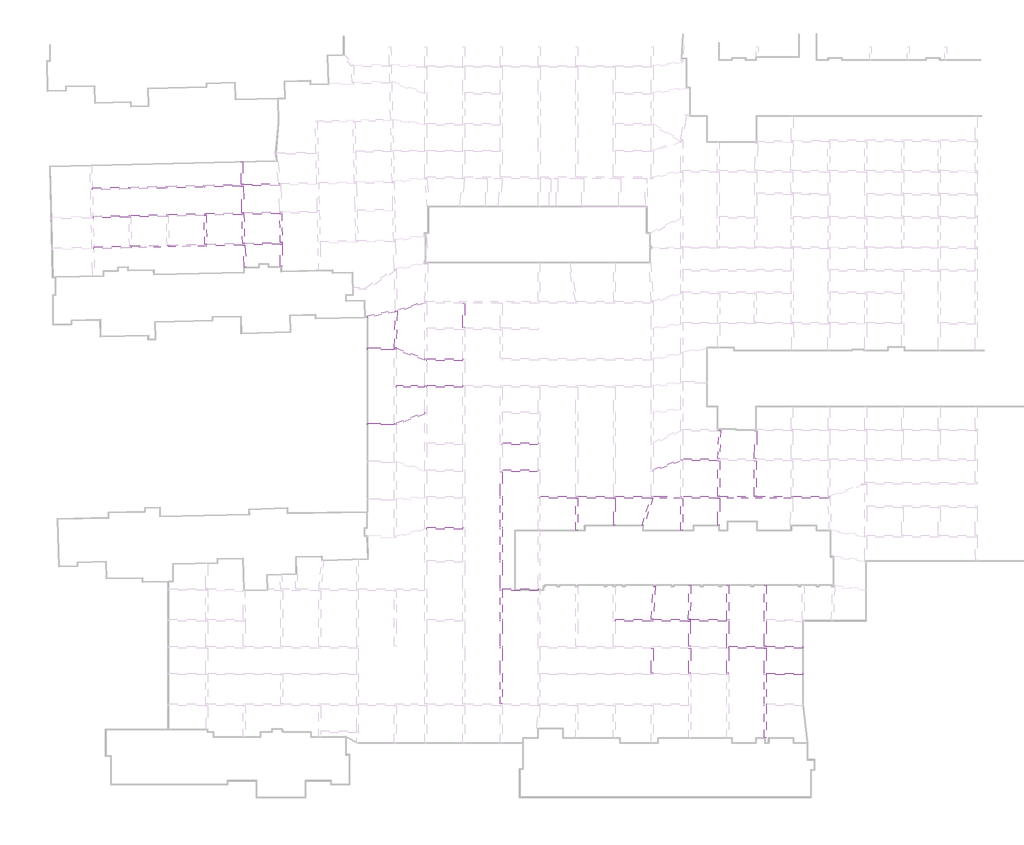
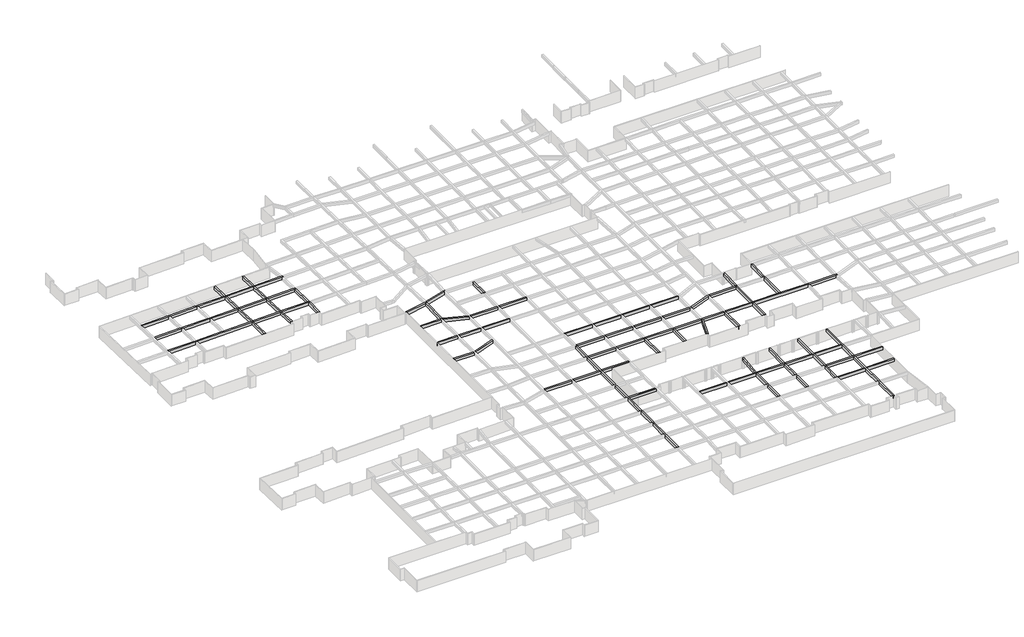
# One storey, part 10 of 20: 51 beams.
"""IFC4 building model written with IfcOpenShell, lengths in millimetres."""

import ifcopenshell
import ifcopenshell.guid

model = None  # the IFC model being written
_history = None  # IfcOwnerHistory: only IFC2X3 demands one
_inside = {}  # id of a spatial element -> (the spatial element, [elements in it])
_under = {}  # id of a project, library or spatial element -> (it, [spatial elements below it])
_declared = {}  # id of a project -> (the project, [libraries it declares])
_typed = {}  # id of a type object -> (the type object, [elements of that type])
_made_of = {}  # id of a material, layer set ... -> (it, [elements and type objects made of it])


def new_model(schema):
    """Start an empty IFC model of exactly this schema.

    Asked for "IFC4X3", IfcOpenShell would pick the latest addendum, in which some entities
    have other attributes; the version numbers below select the first issue.
    IFC2X3 requires an IfcOwnerHistory on every rooted entity: one is made here for all.
    """
    global model, _history
    if schema == "IFC4X3":
        model = ifcopenshell.file(schema_version=(4, 3, 0, 0))
    else:
        model = ifcopenshell.file(schema=schema)
    _inside.clear()
    _under.clear()
    _declared.clear()
    _typed.clear()
    _made_of.clear()
    _history = None
    if model.schema == "IFC2X3":
        org = make("IfcOrganization", Name="unknown")
        user = make(
            "IfcPersonAndOrganization",
            ThePerson=make("IfcPerson", FamilyName="unknown"),
            TheOrganization=org,
        )
        app = make(
            "IfcApplication",
            ApplicationDeveloper=org,
            Version="unknown",
            ApplicationFullName="unknown",
            ApplicationIdentifier="unknown",
        )
        _history = make(
            "IfcOwnerHistory",
            OwningUser=user,
            OwningApplication=app,
            ChangeAction="ADDED",
            CreationDate=0,
        )
    return model


def make(cls, **values):
    """One entity of the class cls with the attributes given. An attribute that is None is left unset."""
    return model.create_entity(
        cls, **{name: value for name, value in values.items() if value is not None}
    )


def rooted(cls, **values):
    """An entity with a GlobalId (a new one), such as an element, a storey or a relation."""
    return make(cls, GlobalId=ifcopenshell.guid.new(), OwnerHistory=_history, **values)


def si_unit(unit_type, name, prefix=None):
    """IfcSIUnit, for example si_unit("LENGTHUNIT", "METRE", prefix="MILLI")."""
    return make("IfcSIUnit", UnitType=unit_type, Prefix=prefix, Name=name)


def assignment(units):
    """IfcUnitAssignment: the units of a project."""
    return None if units is None else make("IfcUnitAssignment", Units=units)


def point(xyz):
    """IfcCartesianPoint."""
    return None if xyz is None else make("IfcCartesianPoint", Coordinates=xyz)


def direction(xyz):
    """IfcDirection."""
    return None if xyz is None else make("IfcDirection", DirectionRatios=xyz)


def frame(location, z_axis=None, x_axis=None):
    """IfcAxis2Placement3D, a coordinate frame: its origin and axes. An axis left out is left unset."""
    return make(
        "IfcAxis2Placement3D",
        Location=point(location),
        Axis=direction(z_axis),
        RefDirection=direction(x_axis),
    )


def origin():
    """The frame at (0, 0, 0) with its axes left unset."""
    return frame((0.0, 0.0, 0.0))


def place(relative_to, where):
    """IfcLocalPlacement: puts the frame where relative to a parent placement (None: the world)."""
    return make(
        "IfcLocalPlacement", PlacementRelTo=relative_to, RelativePlacement=where
    )


def context(
    kind, dimensions, precision=None, world=None, true_north=None, identifier=None
):
    """IfcGeometricRepresentationContext, for example the 3D "Model" context."""
    return make(
        "IfcGeometricRepresentationContext",
        ContextIdentifier=identifier,
        ContextType=kind,
        CoordinateSpaceDimension=dimensions,
        Precision=precision,
        WorldCoordinateSystem=world,
        TrueNorth=true_north,
    )


def project(units=None, contexts=None):
    """IfcProject with its units and contexts."""
    return rooted(
        "IfcProject",
        Name="project",
        RepresentationContexts=contexts,
        UnitsInContext=assignment(units),
    )


def spatial(cls, under=None, at=None, **own):
    """A site, building, storey or space (cls), placed at a placement, below another one or the project."""
    s = rooted(cls, ObjectPlacement=at, **own)
    if under is not None:
        _under.setdefault(under.id(), (under, []))[1].append(s)
    return s


def polyline(points):
    """IfcPolyline through the points."""
    return make("IfcPolyline", Points=[point(p) for p in points])


def outline(outer, holes=None, kind="AREA"):
    """IfcArbitraryClosedProfileDef: a profile drawn as a closed curve; with holes, ...WithVoids."""
    if holes is None:
        return make("IfcArbitraryClosedProfileDef", ProfileType=kind, OuterCurve=outer)
    return make(
        "IfcArbitraryProfileDefWithVoids",
        ProfileType=kind,
        OuterCurve=outer,
        InnerCurves=holes,
    )


def extrude(swept, where, along, depth):
    """IfcExtrudedAreaSolid: the profile swept, set in the frame where, extruded along a direction by depth."""
    return make(
        "IfcExtrudedAreaSolid",
        SweptArea=swept,
        Position=where,
        ExtrudedDirection=direction(along),
        Depth=depth,
    )


def faces_of(points, faces, orient=None, outer=None):
    """IfcFace entities. A face is a list of loops; a loop is a list of indices into points, from 0.

    orient and outer hold one flag for each loop. By default every Orientation is true, the
    first loop of a face is its IfcFaceOuterBound and the others are IfcFaceBound.
    """
    made = []
    for i, loops in enumerate(faces):
        bounds = []
        for j, loop in enumerate(loops):
            is_outer = j == 0 if outer is None else outer[i][j]
            bounds.append(
                make(
                    "IfcFaceOuterBound" if is_outer else "IfcFaceBound",
                    Bound=make("IfcPolyLoop", Polygon=[points[k] for k in loop]),
                    Orientation=True if orient is None else orient[i][j],
                )
            )
        made.append(make("IfcFace", Bounds=bounds))
    return made


def faceted_brep(points, faces, orient=None, outer=None, voids=None):
    """IfcFacetedBrep: a solid bounded by flat faces; with voids (closed shells), ...WithVoids."""
    shared = [point(p) for p in points]
    hull = make("IfcClosedShell", CfsFaces=faces_of(shared, faces, orient, outer))
    if voids is None:
        return make("IfcFacetedBrep", Outer=hull)
    return make(
        "IfcFacetedBrepWithVoids",
        Outer=hull,
        Voids=[
            make(cls, CfsFaces=faces_of(shared, fs, o, b)) for cls, fs, o, b in voids
        ],
    )


def shape(context_of_items, identifier, shape_type, items):
    """IfcShapeRepresentation: the items that make up one representation, for example the "Body"."""
    return make(
        "IfcShapeRepresentation",
        ContextOfItems=context_of_items,
        RepresentationIdentifier=identifier,
        RepresentationType=shape_type,
        Items=items,
    )


def made_of(thing, what):
    """Note that an element or type object is made of a material, layer set ...; save() writes the relation."""
    if what is not None:
        _made_of.setdefault(what.id(), (what, []))[1].append(thing)
    return thing


def element(
    cls,
    number,
    at=None,
    inside=None,
    cuts=None,
    type_object=None,
    material=None,
    context=None,
    identifier="Body",
    shape_type=None,
    held_by="IfcProductDefinitionShape",
    body=None,
    shapes=None,
    **own,
):
    """One element of the class cls, such as IfcWall. Its Tag is "e" and its number.

    at: its placement. inside: the storey or other place that contains it. cuts: it is an
    opening in that element (IfcRelVoidsElement). A single representation is given by context,
    identifier, shape_type and body (its items); several are given by shapes. held_by: the class
    of the entity that holds the representations. save() writes the other relations.
    """
    e = rooted(cls, Tag="e%d" % number, ObjectPlacement=at, **own)
    if body is not None:
        shapes = [shape(context, identifier, shape_type, body)]
    if shapes is not None:
        e.Representation = make(held_by, Representations=shapes)
    if inside is not None:
        _inside.setdefault(inside.id(), (inside, []))[1].append(e)
    if cuts is not None:
        rooted(
            "IfcRelVoidsElement", RelatingBuildingElement=cuts, RelatedOpeningElement=e
        )
    if type_object is not None:
        _typed.setdefault(type_object.id(), (type_object, []))[1].append(e)
    return made_of(e, material)


def aggregate(whole, parts):
    """IfcRelAggregates: a whole, such as a stair, and the parts it consists of."""
    return rooted("IfcRelAggregates", RelatingObject=whole, RelatedObjects=parts)


def save(model, path):
    """Write the relations noted so far, then the file.

    IfcRelAggregates (storeys below a building ...), IfcRelContainedInSpatialStructure (elements
    in a storey), IfcRelDefinesByType, IfcRelAssociatesMaterial and IfcRelDeclares: one each for
    every whole, place, type object, material and project.
    """
    for whole, parts in _under.values():
        aggregate(whole, parts)
    for where, things in _inside.values():
        rooted(
            "IfcRelContainedInSpatialStructure",
            RelatedElements=things,
            RelatingStructure=where,
        )
    for kind, things in _typed.values():
        rooted("IfcRelDefinesByType", RelatedObjects=things, RelatingType=kind)
    for what, things in _made_of.values():
        rooted("IfcRelAssociatesMaterial", RelatedObjects=things, RelatingMaterial=what)
    for by, libraries in _declared.values():
        rooted("IfcRelDeclares", RelatingContext=by, RelatedDefinitions=libraries)
    model.write(path)


model = new_model("IFC4")

# Units and contexts
model_context = context("Model", 3, world=origin())
ifc_project = project(units=[si_unit("LENGTHUNIT", "METRE", prefix="MILLI")], contexts=[model_context])

# Site, building, storey
site = spatial("IfcSite", under=ifc_project)
building = spatial("IfcBuilding", under=site)
storey = spatial("IfcBuildingStorey", under=building, Name="户型图", Elevation=0.0)

# Beams
placement = place(None, origin())
element("IfcBeam", 1, ObjectType="混凝土 - 矩形梁 : KL_beam", at=placement, inside=storey, context=model_context, shape_type="SweptSolid", body=[
    extrude(outline(polyline([(102845.0, 57619.9584924), (102845.0, 58045.6296013), (108750.0, 60194.8738347), (108750.0, 59769.2027257), (102845.0, 57619.9584924)])), frame((0.0, 0.0, 2500.0), z_axis=(0.0, 0.0, 1.0), x_axis=(1.0, 0.0, 0.0)), (0.0, 0.0, 1.0), 800.0),
])
element("IfcBeam", 2, ObjectType="混凝土 - 矩形梁 : KL_beam", at=placement, inside=storey, context=model_context, shape_type="SweptSolid", body=[
    extrude(outline(polyline([(102445.0, 63683.0), (102445.0, 63283.0), (94850.0, 63283.0), (94850.0, 63683.0), (102445.0, 63683.0)])), frame((0.0, 0.0, 2500.0), z_axis=(0.0, 0.0, 1.0), x_axis=(1.0, 0.0, 0.0)), (0.0, 0.0, 1.0), 800.0),
    extrude(outline(polyline([(70850.0, 63283.0), (70850.0, 63683.0), (78450.0, 63683.0), (78450.0, 63283.0), (70850.0, 63283.0)])), frame((0.0, 0.0, 2500.0), z_axis=(0.0, 0.0, 1.0), x_axis=(1.0, 0.0, 0.0)), (0.0, 0.0, 1.0), 800.0),
    extrude(outline(polyline([(78850.0, 63283.0), (78850.0, 63683.0), (86450.0, 63683.0), (86450.0, 63283.0), (78850.0, 63283.0)])), frame((0.0, 0.0, 2500.0), z_axis=(0.0, 0.0, 1.0), x_axis=(1.0, 0.0, 0.0)), (0.0, 0.0, 1.0), 800.0),
    extrude(outline(polyline([(86850.0, 63283.0), (86850.0, 63683.0), (94450.0, 63683.0), (94450.0, 63283.0), (86850.0, 63283.0)])), frame((0.0, 0.0, 2500.0), z_axis=(0.0, 0.0, 1.0), x_axis=(1.0, 0.0, 0.0)), (0.0, 0.0, 1.0), 800.0),
])
element("IfcBeam", 3, ObjectType="混凝土 - 矩形梁 : KL_beam", at=placement, inside=storey, context=model_context, shape_type="SweptSolid", body=[
    extrude(outline(polyline([(102445.0, 57960.0), (102445.0, 57560.0), (94850.0, 57560.0), (94850.0, 57960.0), (102445.0, 57960.0)])), frame((0.0, 0.0, 2500.0), z_axis=(0.0, 0.0, 1.0), x_axis=(1.0, 0.0, 0.0)), (0.0, 0.0, 1.0), 800.0),
    extrude(outline(polyline([(70850.0, 57560.0), (70850.0, 57960.0), (78450.0, 57960.0), (78450.0, 57560.0), (70850.0, 57560.0)])), frame((0.0, 0.0, 2500.0), z_axis=(0.0, 0.0, 1.0), x_axis=(1.0, 0.0, 0.0)), (0.0, 0.0, 1.0), 800.0),
    extrude(outline(polyline([(78850.0, 57560.0), (78850.0, 57960.0), (86450.0, 57960.0), (86450.0, 57560.0), (78850.0, 57560.0)])), frame((0.0, 0.0, 2500.0), z_axis=(0.0, 0.0, 1.0), x_axis=(1.0, 0.0, 0.0)), (0.0, 0.0, 1.0), 800.0),
    extrude(outline(polyline([(86850.0, 57560.0), (86850.0, 57960.0), (94450.0, 57960.0), (94450.0, 57560.0), (86850.0, 57560.0)])), frame((0.0, 0.0, 2500.0), z_axis=(0.0, 0.0, 1.0), x_axis=(1.0, 0.0, 0.0)), (0.0, 0.0, 1.0), 800.0),
])
element("IfcBeam", 4, ObjectType="混凝土 - 矩形梁 : KL_beam", at=placement, inside=storey, context=model_context, shape_type="Brep", body=[
    faceted_brep([(108750.0, 51965.0, 3300.0), (108750.0, 52365.0, 3300.0), (102845.0, 52365.0, 3300.0), (102445.0, 52365.0, 3300.0), (94850.0, 52365.0, 3300.0), (94450.0, 52365.0, 3300.0), (86850.0, 52365.0, 3300.0), (86450.0, 52365.0, 3300.0), (78850.0, 52365.0, 3300.0), (78850.0, 51965.0, 3300.0), (86450.0, 51965.0, 3300.0), (86850.0, 51965.0, 3300.0), (94450.0, 51965.0, 3300.0), (94850.0, 51965.0, 3300.0), (102369.758159, 51965.0, 3300.0), (102790.3267419, 51965.0, 3300.0), (108750.0, 52365.0, 2500.0), (102845.0, 52365.0, 2500.0), (102445.0, 52365.0, 2500.0), (94850.0, 52365.0, 2500.0), (94450.0, 52365.0, 2500.0), (86850.0, 52365.0, 2500.0), (86450.0, 52365.0, 2500.0), (78850.0, 52365.0, 2500.0), (108750.0, 51965.0, 2500.0), (102790.3267419, 51965.0, 2500.0), (102369.758159, 51965.0, 2500.0), (94850.0, 51965.0, 2500.0), (94450.0, 51965.0, 2500.0), (86850.0, 51965.0, 2500.0), (86450.0, 51965.0, 2500.0), (78850.0, 51965.0, 2500.0)], [[[0, 1, 2, 3, 4, 5, 6, 7, 8, 9, 10, 11, 12, 13, 14, 15]], [[1, 16, 17, 18, 19, 20, 21, 22, 23, 8, 7, 6, 5, 4, 3, 2]], [[16, 24, 25, 26, 27, 28, 29, 30, 31, 23, 22, 21, 20, 19, 18, 17]], [[24, 0, 15, 14, 13, 12, 11, 10, 9, 31, 30, 29, 28, 27, 26, 25]], [[1, 0, 24, 16]], [[9, 8, 23, 31]]]),
    faceted_brep([(78450.0, 52365.0, 3300.0), (78450.0, 51965.0, 3300.0), (78450.0, 51965.0, 2500.0), (78450.0, 52365.0, 2500.0), (70850.0, 52365.0, 3300.0), (70850.0, 51965.0, 3300.0), (70850.0, 52365.0, 2500.0), (70850.0, 51965.0, 2500.0)], [[[0, 1, 2, 3]], [[1, 0, 4, 5]], [[0, 3, 6, 4]], [[3, 2, 7, 6]], [[2, 1, 5, 7]], [[5, 4, 6, 7]]]),
])
element("IfcBeam", 5, ObjectType="混凝土 - 矩形梁 : KL_beam", at=placement, inside=storey, context=model_context, shape_type="Brep", body=[
    faceted_brep([(70850.0, 57560.0, 3300.0), (70450.0, 57560.0, 3300.0), (70450.0, 52365.0, 3300.0), (70450.0, 51965.0, 3300.0), (70450.0, 45760.0, 3300.0), (70450.0, 45360.0, 3300.0), (70450.0, 38790.0, 3300.0), (70450.0, 38390.0, 3300.0), (70450.0, 32740.0, 3300.0), (70450.0, 32340.0, 3300.0), (70450.0, 26240.0, 3300.0), (70450.0, 25840.0, 3300.0), (70450.0, 20540.0, 3300.0), (70450.0, 20140.0, 3300.0), (70450.0, 14840.0, 3300.0), (70450.0, 14440.0, 3300.0), (70450.0, 8340.0, 3300.0), (70850.0, 8340.0, 3300.0), (70850.0, 14440.0, 3300.0), (70850.0, 14840.0, 3300.0), (70850.0, 20140.0, 3300.0), (70850.0, 20540.0, 3300.0), (70850.0, 25840.0, 3300.0), (70850.0, 26240.0, 3300.0), (70850.0, 32340.0, 3300.0), (70850.0, 32740.0, 3300.0), (70850.0, 38390.0, 3300.0), (70850.0, 38790.0, 3300.0), (70850.0, 45360.0, 3300.0), (70850.0, 45760.0, 3300.0), (70850.0, 51965.0, 3300.0), (70850.0, 52365.0, 3300.0), (70450.0, 57560.0, 2500.0), (70450.0, 52365.0, 2500.0), (70450.0, 51965.0, 2500.0), (70450.0, 45760.0, 2500.0), (70450.0, 45360.0, 2500.0), (70450.0, 38790.0, 2500.0), (70450.0, 38390.0, 2500.0), (70450.0, 32740.0, 2500.0), (70450.0, 32340.0, 2500.0), (70450.0, 26240.0, 2500.0), (70450.0, 25840.0, 2500.0), (70450.0, 20540.0, 2500.0), (70450.0, 20140.0, 2500.0), (70450.0, 14840.0, 2500.0), (70450.0, 14440.0, 2500.0), (70450.0, 8340.0, 2500.0), (70850.0, 57560.0, 2500.0), (70850.0, 52365.0, 2500.0), (70850.0, 51965.0, 2500.0), (70850.0, 45760.0, 2500.0), (70850.0, 45360.0, 2500.0), (70850.0, 38790.0, 2500.0), (70850.0, 38390.0, 2500.0), (70850.0, 32740.0, 2500.0), (70850.0, 32340.0, 2500.0), (70850.0, 26240.0, 2500.0), (70850.0, 25840.0, 2500.0), (70850.0, 20540.0, 2500.0), (70850.0, 20140.0, 2500.0), (70850.0, 14840.0, 2500.0), (70850.0, 14440.0, 2500.0), (70850.0, 8340.0, 2500.0)], [[[0, 1, 2, 3, 4, 5, 6, 7, 8, 9, 10, 11, 12, 13, 14, 15, 16, 17, 18, 19, 20, 21, 22, 23, 24, 25, 26, 27, 28, 29, 30, 31]], [[1, 32, 33, 34, 35, 36, 37, 38, 39, 40, 41, 42, 43, 44, 45, 46, 47, 16, 15, 14, 13, 12, 11, 10, 9, 8, 7, 6, 5, 4, 3, 2]], [[32, 48, 49, 50, 51, 52, 53, 54, 55, 56, 57, 58, 59, 60, 61, 62, 63, 47, 46, 45, 44, 43, 42, 41, 40, 39, 38, 37, 36, 35, 34, 33]], [[48, 0, 31, 30, 29, 28, 27, 26, 25, 24, 23, 22, 21, 20, 19, 18, 17, 63, 62, 61, 60, 59, 58, 57, 56, 55, 54, 53, 52, 51, 50, 49]], [[1, 0, 48, 32]], [[17, 16, 47, 63]]]),
])
element("IfcBeam", 6, ObjectType="混凝土 - 矩形梁 : KL_beam", at=placement, inside=storey, context=model_context, shape_type="SweptSolid", body=[
    extrude(outline(polyline([(62450.0, 93310.0), (62850.0, 93310.0), (62850.0, 88060.0), (62450.0, 88060.0), (62450.0, 93310.0)])), frame((0.0, 0.0, 2500.0), z_axis=(0.0, 0.0, 1.0), x_axis=(1.0, 0.0, 0.0)), (0.0, 0.0, 1.0), 800.0),
])
element("IfcBeam", 7, ObjectType="混凝土 - 矩形梁 : KL_beam", at=placement, inside=storey, context=model_context, shape_type="SweptSolid", body=[
    extrude(outline(polyline([(54850.0, 81110.0), (54850.0, 81510.0), (62450.0, 81510.0), (62450.0, 81110.0), (54850.0, 81110.0)])), frame((0.0, 0.0, 2500.0), z_axis=(0.0, 0.0, 1.0), x_axis=(1.0, 0.0, 0.0)), (0.0, 0.0, 1.0), 800.0),
    extrude(outline(polyline([(70450.0, 81510.0), (70450.0, 81110.0), (62850.0, 81110.0), (62850.0, 81510.0), (70450.0, 81510.0)])), frame((0.0, 0.0, 2500.0), z_axis=(0.0, 0.0, 1.0), x_axis=(1.0, 0.0, 0.0)), (0.0, 0.0, 1.0), 800.0),
])
element("IfcBeam", 8, ObjectType="混凝土 - 矩形梁 : KL_beam", at=placement, inside=storey, context=model_context, shape_type="SweptSolid", body=[
    extrude(outline(polyline([(62450.0, 75860.0), (62450.0, 75460.0), (54850.0, 75460.0), (54850.0, 75860.0), (62450.0, 75860.0)])), frame((0.0, 0.0, 2500.0), z_axis=(0.0, 0.0, 1.0), x_axis=(1.0, 0.0, 0.0)), (0.0, 0.0, 1.0), 800.0),
])
element("IfcBeam", 9, ObjectType="混凝土 - 矩形梁 : KL_beam", at=placement, inside=storey, context=model_context, shape_type="SweptSolid", body=[
    extrude(outline(polyline([(78450.0, 45760.0), (78450.0, 45360.0), (70850.0, 45360.0), (70850.0, 45760.0), (78450.0, 45760.0)])), frame((0.0, 0.0, 2500.0), z_axis=(0.0, 0.0, 1.0), x_axis=(1.0, 0.0, 0.0)), (0.0, 0.0, 1.0), 800.0),
    extrude(outline(polyline([(54850.0, 45360.0), (54850.0, 45760.0), (62450.0, 45760.0), (62450.0, 45360.0), (54850.0, 45360.0)])), frame((0.0, 0.0, 2500.0), z_axis=(0.0, 0.0, 1.0), x_axis=(1.0, 0.0, 0.0)), (0.0, 0.0, 1.0), 800.0),
    extrude(outline(polyline([(70450.0, 45760.0), (70450.0, 45360.0), (62850.0, 45360.0), (62850.0, 45760.0), (70450.0, 45760.0)])), frame((0.0, 0.0, 2500.0), z_axis=(0.0, 0.0, 1.0), x_axis=(1.0, 0.0, 0.0)), (0.0, 0.0, 1.0), 800.0),
])
element("IfcBeam", 10, ObjectType="混凝土 - 矩形梁 : KL_beam", at=placement, inside=storey, context=model_context, shape_type="Brep", body=[
    faceted_brep([(110728.5214786, 25840.0, 3300.0), (110725.0304656, 26040.0, 3300.0), (110721.5394526, 26240.0, 3300.0), (110328.4605474, 26240.0, 3300.0), (102848.6320497, 26240.0, 3300.0), (102447.6345431, 26240.0, 3300.0), (94845.0, 26240.0, 3300.0), (94845.0, 25840.0, 3300.0), (102434.0, 25840.0, 3300.0), (102834.0, 25840.0, 3300.0), (110328.4605474, 25840.0, 3300.0), (110728.5214786, 25840.0, 2500.0), (94845.0, 25840.0, 2500.0), (102434.0, 25840.0, 2500.0), (102834.0, 25840.0, 2500.0), (110328.4605474, 25840.0, 2500.0), (110721.5394526, 26240.0, 2500.0), (110725.0304656, 26040.0, 2500.0), (94845.0, 26240.0, 2500.0), (102447.6345431, 26240.0, 2500.0), (102848.6320497, 26240.0, 2500.0), (110328.4605474, 26240.0, 2500.0)], [[[0, 1, 2, 3, 4, 5, 6, 7, 8, 9, 10]], [[11, 0, 10, 9, 8, 7, 12, 13, 14, 15]], [[16, 17, 11, 15, 14, 13, 12, 18, 19, 20, 21]], [[2, 16, 21, 20, 19, 18, 6, 5, 4, 3]], [[7, 6, 18, 12]], [[2, 1, 0, 11, 17, 16]]]),
    faceted_brep([(86850.0, 25840.0, 3300.0), (86850.0, 26240.0, 3300.0), (86850.0, 26240.0, 2500.0), (86850.0, 25840.0, 2500.0), (94445.0, 26240.0, 3300.0), (94445.0, 25840.0, 3300.0), (94445.0, 25840.0, 2500.0), (94445.0, 26240.0, 2500.0)], [[[0, 1, 2, 3]], [[4, 5, 6, 7]], [[1, 0, 5, 4]], [[0, 3, 6, 5]], [[3, 2, 7, 6]], [[2, 1, 4, 7]]]),
])
element("IfcBeam", 11, ObjectType="混凝土 - 矩形梁 : KL_beam", at=placement, inside=storey, context=model_context, shape_type="SweptSolid", body=[
    extrude(outline(polyline([(102434.0, 25840.0), (102834.0, 25840.0), (102834.0, 20540.0), (102434.0, 20540.0), (102434.0, 25840.0)])), frame((0.0, 0.0, 2500.0), z_axis=(0.0, 0.0, 1.0), x_axis=(1.0, 0.0, 0.0)), (0.0, 0.0, 1.0), 800.0),
    extrude(outline(polyline([(102834.0, 14840.0), (102434.0, 14840.0), (102434.0, 20140.0), (102834.0, 20140.0), (102834.0, 14840.0)])), frame((0.0, 0.0, 2500.0), z_axis=(0.0, 0.0, 1.0), x_axis=(1.0, 0.0, 0.0)), (0.0, 0.0, 1.0), 800.0),
])
element("IfcBeam", 12, ObjectType="混凝土 - 矩形梁 : KL_beam", at=placement, inside=storey, context=model_context, shape_type="SweptSolid", body=[
    extrude(outline(polyline([(110328.4605474, 25840.0), (110728.5214786, 25840.0), (110821.0333227, 20540.0), (110420.9723915, 20540.0), (110328.4605474, 25840.0)])), frame((0.0, 0.0, 2500.0), z_axis=(0.0, 0.0, 1.0), x_axis=(1.0, 0.0, 0.0)), (0.0, 0.0, 1.0), 800.0),
])
element("IfcBeam", 13, ObjectType="混凝土 - 矩形梁 : KL_beam", at=placement, inside=storey, context=model_context, shape_type="SweptSolid", body=[
    extrude(outline(polyline([(110824.4938701, 14840.0), (110424.4938701, 14840.0), (110424.4938701, 20140.0), (110824.4938701, 20140.0), (110824.4938701, 14840.0)])), frame((0.0, 0.0, 2500.0), z_axis=(0.0, 0.0, 1.0), x_axis=(1.0, 0.0, 0.0)), (0.0, 0.0, 1.0), 800.0),
])
element("IfcBeam", 14, ObjectType="混凝土 - 矩形梁 : KL_beam", at=placement, inside=storey, context=model_context, shape_type="Brep", body=[
    faceted_brep([(118450.0, 33507.0, 3300.0), (118850.0, 33507.0, 3300.0), (118850.0, 33507.0, 2500.0), (118450.0, 33507.0, 2500.0), (118450.0, 26240.0, 3300.0), (118450.0, 25840.0, 3300.0), (118450.0, 20540.0, 3300.0), (118450.0, 20140.0, 3300.0), (118450.0, 14840.0, 3300.0), (118850.0, 14840.0, 3300.0), (118850.0, 20140.0, 3300.0), (118850.0, 20540.0, 3300.0), (118850.0, 25840.0, 3300.0), (118850.0, 26240.0, 3300.0), (118850.0, 14840.0, 2500.0), (118850.0, 20140.0, 2500.0), (118850.0, 20540.0, 2500.0), (118850.0, 25840.0, 2500.0), (118850.0, 26240.0, 2500.0), (118450.0, 14840.0, 2500.0), (118450.0, 20140.0, 2500.0), (118450.0, 20540.0, 2500.0), (118450.0, 25840.0, 2500.0), (118450.0, 26240.0, 2500.0)], [[[0, 1, 2, 3]], [[1, 0, 4, 5, 6, 7, 8, 9, 10, 11, 12, 13]], [[2, 1, 13, 12, 11, 10, 9, 14, 15, 16, 17, 18]], [[3, 2, 18, 17, 16, 15, 14, 19, 20, 21, 22, 23]], [[0, 3, 23, 22, 21, 20, 19, 8, 7, 6, 5, 4]], [[9, 8, 19, 14]]]),
])
element("IfcBeam", 15, ObjectType="混凝土 - 矩形梁 : KL_beam", at=placement, inside=storey, context=model_context, shape_type="Brep", body=[
    faceted_brep([(110454.5273167, 33462.3603793, 3300.0), (110854.4663948, 33455.3794168, 3300.0), (110854.4663948, 33455.3794168, 2500.0), (110454.5273167, 33462.3603793, 2500.0), (110328.4605474, 26240.0, 3300.0), (110721.5394526, 26240.0, 3300.0), (110725.0304656, 26040.0, 3300.0), (110728.5214786, 26240.0, 3300.0), (110725.0304656, 26040.0, 2500.0), (110728.5214786, 26240.0, 2500.0), (110721.5394526, 26240.0, 2500.0), (110328.4605474, 26240.0, 2500.0)], [[[0, 1, 2, 3]], [[1, 0, 4, 5, 6, 7]], [[2, 1, 7, 6, 8, 9]], [[3, 2, 9, 8, 10, 11]], [[0, 3, 11, 4]], [[10, 5, 4, 11]], [[5, 10, 8, 6]]]),
])
element("IfcBeam", 16, ObjectType="混凝土 - 矩形梁 : KL_beam", at=placement, inside=storey, context=model_context, shape_type="SweptSolid", body=[
    extrude(outline(polyline([(102944.4623549, 33270.6006236), (103343.4673297, 33242.4043457), (102848.6320497, 26240.0), (102447.6345431, 26240.0), (102944.4623549, 33270.6006236)])), frame((0.0, 0.0, 2500.0), z_axis=(0.0, 0.0, 1.0), x_axis=(1.0, 0.0, 0.0)), (0.0, 0.0, 1.0), 800.0),
])
element("IfcBeam", 17, ObjectType="混凝土 - 矩形梁 : KL_beam", at=placement, inside=storey, context=model_context, shape_type="SweptSolid", body=[
    extrude(outline(polyline([(110728.5214786, 25840.0), (110725.0304656, 26040.0), (110728.5214786, 26240.0), (118450.0, 26240.0), (118450.0, 25840.0), (110728.5214786, 25840.0)])), frame((0.0, 0.0, 2500.0), z_axis=(0.0, 0.0, 1.0), x_axis=(1.0, 0.0, 0.0)), (0.0, 0.0, 1.0), 800.0),
    extrude(outline(polyline([(118850.0, 25840.0), (118850.0, 26240.0), (126444.0, 26240.0), (126444.0, 25840.0), (118850.0, 25840.0)])), frame((0.0, 0.0, 2500.0), z_axis=(0.0, 0.0, 1.0), x_axis=(1.0, 0.0, 0.0)), (0.0, 0.0, 1.0), 800.0),
])
element("IfcBeam", 18, ObjectType="混凝土 - 矩形梁 : KL_beam", at=placement, inside=storey, context=model_context, shape_type="Brep", body=[
    faceted_brep([(126844.0, 33507.0, 3300.0), (126844.0, 33507.0, 2500.0), (126444.0, 33507.0, 2500.0), (126444.0, 33507.0, 3300.0), (126444.0, 26240.0, 3300.0), (126444.0, 25840.0, 3300.0), (126444.0, 20540.0, 3300.0), (126844.0, 20540.0, 3300.0), (126844.0, 25837.4184717, 3300.0), (126844.0, 26237.453407, 3300.0), (126444.0, 26240.0, 2500.0), (126444.0, 25840.0, 2500.0), (126444.0, 20540.0, 2500.0), (126844.0, 26237.453407, 2500.0), (126844.0, 25837.4184717, 2500.0), (126844.0, 20540.0, 2500.0)], [[[0, 1, 2, 3]], [[0, 3, 4, 5, 6, 7, 8, 9]], [[3, 2, 10, 11, 12, 6, 5, 4]], [[2, 1, 13, 14, 15, 12, 11, 10]], [[1, 0, 9, 8, 7, 15, 14, 13]], [[7, 6, 12, 15]]]),
])
element("IfcBeam", 19, ObjectType="混凝土 - 矩形梁 : KL_beam", at=placement, inside=storey, context=model_context, shape_type="Brep", body=[
    faceted_brep([(134623.3674306, 20540.0, 3300.0), (134623.3674306, 20140.0, 3300.0), (134623.3674306, 20140.0, 2500.0), (134623.3674306, 20540.0, 2500.0), (126844.0, 20540.0, 3300.0), (126444.0, 20540.0, 3300.0), (118850.0, 20540.0, 3300.0), (118850.0, 20140.0, 3300.0), (126444.0, 20140.0, 3300.0), (126844.0, 20140.0, 3300.0), (118850.0, 20140.0, 2500.0), (126444.0, 20140.0, 2500.0), (126844.0, 20140.0, 2500.0), (118850.0, 20540.0, 2500.0), (126444.0, 20540.0, 2500.0), (126844.0, 20540.0, 2500.0)], [[[0, 1, 2, 3]], [[1, 0, 4, 5, 6, 7, 8, 9]], [[2, 1, 9, 8, 7, 10, 11, 12]], [[3, 2, 12, 11, 10, 13, 14, 15]], [[0, 3, 15, 14, 13, 6, 5, 4]], [[7, 6, 13, 10]]]),
])
element("IfcBeam", 20, ObjectType="混凝土 - 矩形梁 : KL_beam", at=placement, inside=storey, context=model_context, shape_type="Brep", body=[
    faceted_brep([(126844.0, 1106.0, 3300.0), (126444.0, 1106.0, 3300.0), (126444.0, 1106.0, 2500.0), (126844.0, 1106.0, 2500.0), (126844.0, 7940.0, 3300.0), (126844.0, 8340.0, 3300.0), (126844.0, 14440.0, 3300.0), (126844.0, 14840.0, 3300.0), (126844.0, 20140.0, 3300.0), (126444.0, 20140.0, 3300.0), (126444.0, 14840.0, 3300.0), (126444.0, 14440.0, 3300.0), (126444.0, 8340.0, 3300.0), (126444.0, 7940.0, 3300.0), (126444.0, 20140.0, 2500.0), (126444.0, 14840.0, 2500.0), (126444.0, 14440.0, 2500.0), (126444.0, 8340.0, 2500.0), (126444.0, 7940.0, 2500.0), (126844.0, 20140.0, 2500.0), (126844.0, 14840.0, 2500.0), (126844.0, 14440.0, 2500.0), (126844.0, 8340.0, 2500.0), (126844.0, 7940.0, 2500.0)], [[[0, 1, 2, 3]], [[1, 0, 4, 5, 6, 7, 8, 9, 10, 11, 12, 13]], [[2, 1, 13, 12, 11, 10, 9, 14, 15, 16, 17, 18]], [[3, 2, 18, 17, 16, 15, 14, 19, 20, 21, 22, 23]], [[0, 3, 23, 22, 21, 20, 19, 8, 7, 6, 5, 4]], [[9, 8, 19, 14]]]),
])
element("IfcBeam", 21, ObjectType="混凝土 - 矩形梁 : KL_beam", at=placement, inside=storey, context=model_context, shape_type="SweptSolid", body=[
    extrude(outline(polyline([(134623.3674306, 14840.0), (134623.3674306, 14440.0), (126844.0, 14440.0), (126844.0, 14840.0), (134623.3674306, 14840.0)])), frame((0.0, 0.0, 2500.0), z_axis=(0.0, 0.0, 1.0), x_axis=(1.0, 0.0, 0.0)), (0.0, 0.0, 1.0), 800.0),
    extrude(outline(polyline([(118850.0, 14440.0), (118850.0, 14840.0), (126444.0, 14840.0), (126444.0, 14440.0), (118850.0, 14440.0)])), frame((0.0, 0.0, 2500.0), z_axis=(0.0, 0.0, 1.0), x_axis=(1.0, 0.0, 0.0)), (0.0, 0.0, 1.0), 800.0),
])
element("IfcBeam", 22, ObjectType="混凝土 - 矩形梁 : KL_beam", at=placement, inside=storey, context=model_context, shape_type="Brep", body=[
    faceted_brep([(48350.0, 83800.3620102, 3300.0), (48350.0, 83375.0226052, 3300.0), (54450.0, 81169.6379898, 3300.0), (54450.0, 81594.9773948, 3300.0), (48353.8968226, 83798.953159, 3300.0), (48350.0, 83375.0226052, 2500.0), (54450.0, 81169.6379898, 2500.0), (48350.0, 83800.3620102, 2500.0), (48353.8968226, 83798.953159, 2500.0), (54450.0, 81594.9773948, 2500.0)], [[[0, 1, 2, 3, 4]], [[1, 5, 6, 2]], [[5, 7, 8, 9, 6]], [[7, 0, 4, 3, 9, 8]], [[1, 0, 7, 5]], [[3, 2, 6, 9]]]),
])
element("IfcBeam", 23, ObjectType="混凝土 - 矩形梁 : KL_beam", at=placement, inside=storey, context=model_context, shape_type="SweptSolid", body=[
    extrude(outline(polyline([(42250.0, 75460.0), (42250.0, 75860.0), (47950.0, 75860.0), (47950.0, 75460.0), (42250.0, 75460.0)])), frame((0.0, 0.0, 2500.0), z_axis=(0.0, 0.0, 1.0), x_axis=(1.0, 0.0, 0.0)), (0.0, 0.0, 1.0), 800.0),
    extrude(outline(polyline([(54450.0, 75860.0), (54450.0, 75460.0), (48350.0, 75460.0), (48350.0, 75860.0), (54450.0, 75860.0)])), frame((0.0, 0.0, 2500.0), z_axis=(0.0, 0.0, 1.0), x_axis=(1.0, 0.0, 0.0)), (0.0, 0.0, 1.0), 800.0),
])
element("IfcBeam", 24, ObjectType="混凝土 - 矩形梁 : KL_beam", at=placement, inside=storey, context=model_context, shape_type="SweptSolid", body=[
    extrude(outline(polyline([(42250.0, 67460.0), (42250.0, 67860.0), (47950.0, 67860.0), (47950.0, 67460.0), (42250.0, 67460.0)])), frame((0.0, 0.0, 2500.0), z_axis=(0.0, 0.0, 1.0), x_axis=(1.0, 0.0, 0.0)), (0.0, 0.0, 1.0), 800.0),
])
element("IfcBeam", 25, ObjectType="混凝土 - 矩形梁 : KL_beam", at=placement, inside=storey, context=model_context, shape_type="SweptSolid", body=[
    extrude(outline(polyline([(54450.0, 70165.8480304), (54450.0, 69740.1769214), (48350.0, 67519.9584924), (48350.0, 67945.6296013), (54450.0, 70165.8480304)])), frame((0.0, 0.0, 2500.0), z_axis=(0.0, 0.0, 1.0), x_axis=(1.0, 0.0, 0.0)), (0.0, 0.0, 1.0), 800.0),
])
element("IfcBeam", 26, ObjectType="混凝土 - 矩形梁 : KL_beam", at=placement, inside=storey, context=model_context, shape_type="SweptSolid", body=[
    extrude(outline(polyline([(70850.0, 32340.0), (70850.0, 32740.0), (78450.0, 32740.0), (78450.0, 32340.0), (70850.0, 32340.0)])), frame((0.0, 0.0, 2500.0), z_axis=(0.0, 0.0, 1.0), x_axis=(1.0, 0.0, 0.0)), (0.0, 0.0, 1.0), 800.0),
])
element("IfcBeam", 27, ObjectType="混凝土 - 矩形梁 : KL_beam", at=placement, inside=storey, context=model_context, shape_type="SweptSolid", body=[
    extrude(outline(polyline([(86850.0, 45098.6250189), (86450.0, 45098.6250189), (86450.0, 51965.0), (86850.0, 51965.0), (86850.0, 45098.6250189)])), frame((0.0, 0.0, 2500.0), z_axis=(0.0, 0.0, 1.0), x_axis=(1.0, 0.0, 0.0)), (0.0, 0.0, 1.0), 800.0),
])
element("IfcBeam", 28, ObjectType="混凝土 - 矩形梁 : KL_beam", at=placement, inside=storey, context=model_context, shape_type="SweptSolid", body=[
    extrude(outline(polyline([(94850.0, 46158.0), (94450.0, 46158.0), (94450.0, 51965.0), (94850.0, 51965.0), (94850.0, 46158.0)])), frame((0.0, 0.0, 2500.0), z_axis=(0.0, 0.0, 1.0), x_axis=(1.0, 0.0, 0.0)), (0.0, 0.0, 1.0), 800.0),
])
element("IfcBeam", 29, ObjectType="混凝土 - 矩形梁 : KL_beam", at=placement, inside=storey, context=model_context, shape_type="SweptSolid", body=[
    extrude(outline(polyline([(100884.3559387, 46096.6419196), (100503.9185821, 46220.2033118), (102369.758159, 51965.0), (102790.3267419, 51965.0), (100884.3559387, 46096.6419196)])), frame((0.0, 0.0, 2500.0), z_axis=(0.0, 0.0, 1.0), x_axis=(1.0, 0.0, 0.0)), (0.0, 0.0, 1.0), 800.0),
])
element("IfcBeam", 30, ObjectType="混凝土 - 矩形梁 : KL_beam", at=placement, inside=storey, context=model_context, shape_type="SweptSolid", body=[
    extrude(outline(polyline([(109150.0, 45108.0), (108750.0, 45108.0), (108750.0, 51965.0), (109150.0, 51965.0), (109150.0, 45108.0)])), frame((0.0, 0.0, 2500.0), z_axis=(0.0, 0.0, 1.0), x_axis=(1.0, 0.0, 0.0)), (0.0, 0.0, 1.0), 800.0),
])
element("IfcBeam", 31, ObjectType="混凝土 - 矩形梁 : KL_beam", at=placement, inside=storey, context=model_context, shape_type="Brep", body=[
    faceted_brep([(140350.0, 51965.0, 3300.0), (140350.0, 52026.3999064, 3300.0), (140350.0, 52365.0, 3300.0), (139950.0, 52365.0, 3300.0), (132511.0, 52365.0, 3300.0), (132111.0, 52365.0, 3300.0), (124740.0498394, 52365.0, 3300.0), (124340.0498394, 52365.0, 3300.0), (116950.0, 52365.0, 3300.0), (116550.0, 52365.0, 3300.0), (109150.0, 52365.0, 3300.0), (109150.0, 51965.0, 3300.0), (116550.0, 51965.0, 3300.0), (116950.0, 51965.0, 3300.0), (132105.4993808, 51965.0, 3300.0), (132505.6466155, 51965.0, 3300.0), (139958.0768904, 51965.0, 3300.0), (140186.2669164, 51965.0, 3300.0), (140350.0, 51965.0, 2500.0), (109150.0, 51965.0, 2500.0), (116550.0, 51965.0, 2500.0), (116950.0, 51965.0, 2500.0), (132105.4993808, 51965.0, 2500.0), (132505.6466155, 51965.0, 2500.0), (139958.0768904, 51965.0, 2500.0), (140186.2669164, 51965.0, 2500.0), (140350.0, 52365.0, 2500.0), (140350.0, 52026.3999064, 2500.0), (109150.0, 52365.0, 2500.0), (116550.0, 52365.0, 2500.0), (116950.0, 52365.0, 2500.0), (124340.0498394, 52365.0, 2500.0), (124740.0498394, 52365.0, 2500.0), (132111.0, 52365.0, 2500.0), (132511.0, 52365.0, 2500.0), (139950.0, 52365.0, 2500.0)], [[[0, 1, 2, 3, 4, 5, 6, 7, 8, 9, 10, 11, 12, 13, 14, 15, 16, 17]], [[18, 0, 17, 16, 15, 14, 13, 12, 11, 19, 20, 21, 22, 23, 24, 25]], [[26, 27, 18, 25, 24, 23, 22, 21, 20, 19, 28, 29, 30, 31, 32, 33, 34, 35]], [[2, 26, 35, 34, 33, 32, 31, 30, 29, 28, 10, 9, 8, 7, 6, 5, 4, 3]], [[11, 10, 28, 19]], [[2, 1, 0, 18, 27, 26]]]),
])
element("IfcBeam", 32, ObjectType="混凝土 - 矩形梁 : KL_beam", at=placement, inside=storey, context=model_context, shape_type="SweptSolid", body=[
    extrude(outline(polyline([(124446.4785214, 66190.0), (124846.5394526, 66190.0), (124743.5545695, 60290.0), (124343.4936383, 60290.0), (124446.4785214, 66190.0)])), frame((0.0, 0.0, 2500.0), z_axis=(0.0, 0.0, 1.0), x_axis=(1.0, 0.0, 0.0)), (0.0, 0.0, 1.0), 800.0),
])
element("IfcBeam", 33, ObjectType="混凝土 - 矩形梁 : KL_beam", at=placement, inside=storey, context=model_context, shape_type="SweptSolid", body=[
    extrude(outline(polyline([(124740.0498394, 52365.0), (124340.0498394, 52365.0), (124340.0498394, 59890.0), (124740.0498394, 59890.0), (124740.0498394, 52365.0)])), frame((0.0, 0.0, 2500.0), z_axis=(0.0, 0.0, 1.0), x_axis=(1.0, 0.0, 0.0)), (0.0, 0.0, 1.0), 800.0),
])
element("IfcBeam", 34, ObjectType="混凝土 - 矩形梁 : KL_beam", at=placement, inside=storey, context=model_context, shape_type="Brep", body=[
    faceted_brep([(109150.0, 60254.832327, 3300.0), (109150.0, 59854.832327, 3300.0), (116550.0, 59854.832327, 3300.0), (116550.0, 59890.0, 3300.0), (116550.0, 60254.832327, 3300.0), (109150.0, 59854.832327, 2500.0), (116550.0, 59854.832327, 2500.0), (109150.0, 60254.832327, 2500.0), (116550.0, 60254.832327, 2500.0), (116550.0, 59890.0, 2500.0)], [[[0, 1, 2, 3, 4]], [[1, 5, 6, 2]], [[5, 7, 8, 9, 6]], [[7, 0, 4, 8]], [[1, 0, 7, 5]], [[2, 6, 9, 8, 4, 3]]]),
])
element("IfcBeam", 35, ObjectType="混凝土 - 矩形梁 : KL_beam", at=placement, inside=storey, context=model_context, shape_type="Brep", body=[
    faceted_brep([(116950.0, 59890.0, 3300.0), (116550.0, 59890.0, 3300.0), (116550.0, 59854.832327, 3300.0), (116550.0, 52365.0, 3300.0), (116950.0, 52365.0, 3300.0), (116550.0, 59890.0, 2500.0), (116550.0, 59854.832327, 2500.0), (116550.0, 52365.0, 2500.0), (116950.0, 59890.0, 2500.0), (116950.0, 52365.0, 2500.0)], [[[0, 1, 2, 3, 4]], [[1, 5, 6, 7, 3, 2]], [[5, 8, 9, 7, 6]], [[8, 0, 4, 9]], [[1, 0, 8, 5]], [[4, 3, 7, 9]]]),
])
element("IfcBeam", 36, ObjectType="混凝土 - 矩形梁 : KL_beam", at=placement, inside=storey, context=model_context, shape_type="SweptSolid", body=[
    extrude(outline(polyline([(116777.125435, 66350.0834765), (117176.865054, 66335.6530576), (116958.6197216, 60290.0), (116558.359171, 60290.0), (116777.125435, 66350.0834765)])), frame((0.0, 0.0, 2500.0), z_axis=(0.0, 0.0, 1.0), x_axis=(1.0, 0.0, 0.0)), (0.0, 0.0, 1.0), 800.0),
])
element("IfcBeam", 37, ObjectType="混凝土 - 矩形梁 : KL_beam", at=placement, inside=storey, context=model_context, shape_type="SweptSolid", body=[
    extrude(outline(polyline([(116950.0, 46158.0), (116550.0, 46158.0), (116550.0, 51965.0), (116950.0, 51965.0), (116950.0, 46158.0)])), frame((0.0, 0.0, 2500.0), z_axis=(0.0, 0.0, 1.0), x_axis=(1.0, 0.0, 0.0)), (0.0, 0.0, 1.0), 800.0),
])
element("IfcBeam", 38, ObjectType="混凝土 - 矩形梁 : KL_beam", at=placement, inside=storey, context=model_context, shape_type="Brep", body=[
    faceted_brep([(23898.6430493, 118293.3689104, 3300.0), (23889.0031982, 118693.2527351, 3300.0), (23486.6252708, 118683.5527596, 3300.0), (15906.1264471, 118500.8124843, 3300.0), (15506.2426223, 118491.1726332, 3300.0), (7877.4113984, 118307.2672267, 3300.0), (7477.5275736, 118297.6273756, 3300.0), (-120.335014, 118114.4685185, 3300.0), (-520.2188388, 118104.8286674, 3300.0), (-8079.7847303, 117922.5930146, 3300.0), (-8479.6685551, 117912.9531635, 3300.0), (-16078.8028638, 117729.7636495, 3300.0), (-16069.1557852, 117329.879999, 3300.0), (-8470.0214764, 117513.069513, 3300.0), (-8070.1376517, 117522.7093641, 3300.0), (-510.577611, 117704.9448759, 3300.0), (-110.6937863, 117714.584727, 3300.0), (7487.1746523, 117897.7437251, 3300.0), (7887.0584771, 117907.3835762, 3300.0), (15511.553025, 118091.1844401, 3300.0), (15911.4368497, 118100.8242912, 3300.0), (23519.8781337, 118284.238165, 3300.0), (23898.6430493, 118293.3689104, 2500.0), (-16069.1557852, 117329.879999, 2500.0), (-8470.0214764, 117513.069513, 2500.0), (-8070.1376517, 117522.7093641, 2500.0), (-510.577611, 117704.9448759, 2500.0), (-110.6937863, 117714.584727, 2500.0), (7487.1746523, 117897.7437251, 2500.0), (7887.0584771, 117907.3835762, 2500.0), (15511.553025, 118091.1844401, 2500.0), (15911.4368497, 118100.8242912, 2500.0), (23519.8781337, 118284.238165, 2500.0), (23889.0031982, 118693.2527351, 2500.0), (-16078.8028638, 117729.7636495, 2500.0), (-8479.6685551, 117912.9531635, 2500.0), (-8079.7847303, 117922.5930146, 2500.0), (-520.2188388, 118104.8286674, 2500.0), (-120.335014, 118114.4685185, 2500.0), (7477.5275736, 118297.6273756, 2500.0), (7877.4113984, 118307.2672267, 2500.0), (15506.2426223, 118491.1726332, 2500.0), (15906.1264471, 118500.8124843, 2500.0), (23486.6252708, 118683.5527596, 2500.0)], [[[0, 1, 2, 3, 4, 5, 6, 7, 8, 9, 10, 11, 12, 13, 14, 15, 16, 17, 18, 19, 20, 21]], [[22, 0, 21, 20, 19, 18, 17, 16, 15, 14, 13, 12, 23, 24, 25, 26, 27, 28, 29, 30, 31, 32]], [[33, 22, 32, 31, 30, 29, 28, 27, 26, 25, 24, 23, 34, 35, 36, 37, 38, 39, 40, 41, 42, 43]], [[1, 33, 43, 42, 41, 40, 39, 38, 37, 36, 35, 34, 11, 10, 9, 8, 7, 6, 5, 4, 3, 2]], [[12, 11, 34, 23]], [[1, 0, 22, 33]]]),
])
element("IfcBeam", 39, ObjectType="混凝土 - 矩形梁 : KL_beam", at=placement, inside=storey, context=model_context, shape_type="Brep", body=[
    faceted_brep([(24064.3808816, 112294.8930572, 3300.0), (24054.7407895, 112694.7768761, 3300.0), (23654.8569706, 112685.136784, 3300.0), (16046.4157971, 112501.7183262, 3300.0), (15646.5319782, 112492.0782341, 3300.0), (8022.1353664, 112308.2751349, 3300.0), (7622.2515474, 112298.6350428, 3300.0), (24.3012959, 112115.4694921, 3300.0), (-375.582523, 112105.8294, 3300.0), (-7935.0605304, 111923.5913086, 3300.0), (-8334.9443493, 111913.9512165, 3300.0), (-15934.0785476, 111730.7571241, 3300.0), (-15924.4314689, 111330.8734737, 3300.0), (-8325.2972707, 111514.0675661, 3300.0), (-7925.4134517, 111523.7076581, 3300.0), (-365.9412952, 111705.9456085, 3300.0), (33.9425237, 111715.5857005, 3300.0), (7631.8986261, 111898.7513923, 3300.0), (8031.7824451, 111908.3914844, 3300.0), (15648.2195155, 112092.0027011, 3300.0), (16048.1033344, 112101.6427932, 3300.0), (23664.4970627, 112285.2529651, 3300.0), (24064.3808816, 112294.8930572, 2500.0), (-15924.4314689, 111330.8734737, 2500.0), (-8325.2972707, 111514.0675661, 2500.0), (-7925.4134517, 111523.7076581, 2500.0), (-365.9412952, 111705.9456085, 2500.0), (33.9425237, 111715.5857005, 2500.0), (7631.8986261, 111898.7513923, 2500.0), (8031.7824451, 111908.3914844, 2500.0), (15648.2195155, 112092.0027011, 2500.0), (16048.1033344, 112101.6427932, 2500.0), (23664.4970627, 112285.2529651, 2500.0), (24054.7407895, 112694.7768761, 2500.0), (-15934.0785476, 111730.7571241, 2500.0), (-8334.9443493, 111913.9512165, 2500.0), (-7935.0605304, 111923.5913086, 2500.0), (-375.582523, 112105.8294, 2500.0), (24.3012959, 112115.4694921, 2500.0), (7622.2515474, 112298.6350428, 2500.0), (8022.1353664, 112308.2751349, 2500.0), (15646.5319782, 112492.0782341, 2500.0), (16046.4157971, 112501.7183262, 2500.0), (23654.8569706, 112685.136784, 2500.0)], [[[0, 1, 2, 3, 4, 5, 6, 7, 8, 9, 10, 11, 12, 13, 14, 15, 16, 17, 18, 19, 20, 21]], [[22, 0, 21, 20, 19, 18, 17, 16, 15, 14, 13, 12, 23, 24, 25, 26, 27, 28, 29, 30, 31, 32]], [[33, 22, 32, 31, 30, 29, 28, 27, 26, 25, 24, 23, 34, 35, 36, 37, 38, 39, 40, 41, 42, 43]], [[1, 33, 43, 42, 41, 40, 39, 38, 37, 36, 35, 34, 11, 10, 9, 8, 7, 6, 5, 4, 3, 2]], [[12, 11, 34, 23]], [[1, 0, 22, 33]]]),
])
element("IfcBeam", 40, ObjectType="混凝土 - 矩形梁 : KL_beam", at=placement, inside=storey, context=model_context, shape_type="Brep", body=[
    faceted_brep([(24221.0298802, 105796.8845955, 3300.0), (24216.2679247, 105994.416832, 3300.0), (24211.3897881, 106196.7684144, 3300.0), (23811.5059692, 106187.1283223, 3300.0), (16195.1122409, 106003.5181504, 3300.0), (15795.228422, 105993.8780584, 3300.0), (8178.8978956, 105810.2694101, 3300.0), (7779.0140766, 105800.629318, 3300.0), (180.9687495, 105617.4614753, 3300.0), (-218.9150694, 105607.8213832, 3300.0), (-7778.2980012, 105425.5855838, 3300.0), (-8178.1818202, 105415.9454918, 3300.0), (-15777.3160184, 105232.7513994, 3300.0), (-15767.6689398, 104832.8677489, 3300.0), (-8168.5347415, 105016.0618413, 3300.0), (-7768.6509225, 105025.7019334, 3300.0), (7788.6611553, 105400.7456676, 3300.0), (8188.5449742, 105410.3857596, 3300.0), (15847.3002968, 105595.0171523, 3300.0), (16247.6022502, 105604.6673244, 3300.0), (23816.2679247, 105787.1269051, 3300.0), (24216.2679247, 105796.7697979, 3300.0), (24221.0298802, 105796.8845955, 2500.0), (-15767.6689398, 104832.8677489, 2500.0), (-8168.5347415, 105016.0618413, 2500.0), (-7768.6509225, 105025.7019334, 2500.0), (7788.6611553, 105400.7456676, 2500.0), (8188.5449742, 105410.3857596, 2500.0), (15847.3002968, 105595.0171523, 2500.0), (16247.6022502, 105604.6673244, 2500.0), (23816.2679247, 105787.1269051, 2500.0), (24216.2679247, 105796.7697979, 2500.0), (24211.3897881, 106196.7684144, 2500.0), (24216.2679247, 105994.416832, 2500.0), (-15777.3160184, 105232.7513994, 2500.0), (-8178.1818202, 105415.9454918, 2500.0), (-7778.2980012, 105425.5855838, 2500.0), (-218.9150694, 105607.8213832, 2500.0), (180.9687495, 105617.4614753, 2500.0), (7779.0140766, 105800.629318, 2500.0), (8178.8978956, 105810.2694101, 2500.0), (15795.228422, 105993.8780584, 2500.0), (16195.1122409, 106003.5181504, 2500.0), (23811.5059692, 106187.1283223, 2500.0)], [[[0, 1, 2, 3, 4, 5, 6, 7, 8, 9, 10, 11, 12, 13, 14, 15, 16, 17, 18, 19, 20, 21]], [[22, 0, 21, 20, 19, 18, 17, 16, 15, 14, 13, 23, 24, 25, 26, 27, 28, 29, 30, 31]], [[32, 33, 22, 31, 30, 29, 28, 27, 26, 25, 24, 23, 34, 35, 36, 37, 38, 39, 40, 41, 42, 43]], [[2, 32, 43, 42, 41, 40, 39, 38, 37, 36, 35, 34, 12, 11, 10, 9, 8, 7, 6, 5, 4, 3]], [[13, 12, 34, 23]], [[2, 1, 0, 22, 33, 32]]]),
])
element("IfcBeam", 41, ObjectType="混凝土 - 矩形梁 : KL_beam", at=placement, inside=storey, context=model_context, shape_type="SweptSolid", body=[
    extrude(outline(polyline([(7362.2539331, 123075.8660271), (7762.1375835, 123085.5131058), (7877.4113984, 118307.2672267), (7477.5275736, 118297.6273756), (7362.2539331, 123075.8660271)])), frame((0.0, 0.0, 2500.0), z_axis=(0.0, 0.0, 1.0), x_axis=(1.0, 0.0, 0.0)), (0.0, 0.0, 1.0), 800.0),
    extrude(outline(polyline([(7487.1746523, 117897.7437251), (7887.0584771, 117907.3835762), (8022.1353664, 112308.2751349), (7622.2515474, 112298.6350428), (7487.1746523, 117897.7437251)])), frame((0.0, 0.0, 2500.0), z_axis=(0.0, 0.0, 1.0), x_axis=(1.0, 0.0, 0.0)), (0.0, 0.0, 1.0), 800.0),
    extrude(outline(polyline([(8326.6931089, 99683.9703047), (7926.8094585, 99674.323226), (7788.6611553, 105400.7456676), (8188.5449742, 105410.3857596), (8326.6931089, 99683.9703047)])), frame((0.0, 0.0, 2500.0), z_axis=(0.0, 0.0, 1.0), x_axis=(1.0, 0.0, 0.0)), (0.0, 0.0, 1.0), 800.0),
    extrude(outline(polyline([(7631.8986261, 111898.7513923), (8031.7824451, 111908.3914844), (8178.8978956, 105810.2694101), (7779.0140766, 105800.629318), (7631.8986261, 111898.7513923)])), frame((0.0, 0.0, 2500.0), z_axis=(0.0, 0.0, 1.0), x_axis=(1.0, 0.0, 0.0)), (0.0, 0.0, 1.0), 800.0),
])
element("IfcBeam", 42, ObjectType="混凝土 - 矩形梁 : KL_beam", at=placement, inside=storey, context=model_context, shape_type="SweptSolid", body=[
    extrude(outline(polyline([(16577.7905011, 100882.755347), (16177.4890362, 100873.0981886), (15847.3002968, 105595.0171523), (16247.6022502, 105604.6673244), (16577.7905011, 100882.755347)])), frame((0.0, 0.0, 2500.0), z_axis=(0.0, 0.0, 1.0), x_axis=(1.0, 0.0, 0.0)), (0.0, 0.0, 1.0), 800.0),
])
element("IfcBeam", 43, ObjectType="混凝土 - 矩形梁 : KL_beam", at=placement, inside=storey, context=model_context, shape_type="SweptSolid", body=[
    extrude(outline(polyline([(15648.2195155, 112092.0027011), (16048.1033344, 112101.6427932), (16195.1122409, 106003.5181504), (15795.228422, 105993.8780584), (15648.2195155, 112092.0027011)])), frame((0.0, 0.0, 2500.0), z_axis=(0.0, 0.0, 1.0), x_axis=(1.0, 0.0, 0.0)), (0.0, 0.0, 1.0), 800.0),
])
element("IfcBeam", 44, ObjectType="混凝土 - 矩形梁 : KL_beam", at=placement, inside=storey, context=model_context, shape_type="SweptSolid", body=[
    extrude(outline(polyline([(15511.553025, 118091.1844401), (15911.4368497, 118100.8242912), (16046.4157971, 112501.7183262), (15646.5319782, 112492.0782341), (15511.553025, 118091.1844401)])), frame((0.0, 0.0, 2500.0), z_axis=(0.0, 0.0, 1.0), x_axis=(1.0, 0.0, 0.0)), (0.0, 0.0, 1.0), 800.0),
])
element("IfcBeam", 45, ObjectType="混凝土 - 矩形梁 : KL_beam", at=placement, inside=storey, context=model_context, shape_type="SweptSolid", body=[
    extrude(outline(polyline([(15391.0628579, 123268.9821966), (15790.9466768, 123278.6222886), (15906.1264471, 118500.8124843), (15506.2426223, 118491.1726332), (15391.0628579, 123268.9821966)])), frame((0.0, 0.0, 2500.0), z_axis=(0.0, 0.0, 1.0), x_axis=(1.0, 0.0, 0.0)), (0.0, 0.0, 1.0), 800.0),
])
element("IfcBeam", 46, ObjectType="混凝土 - 矩形梁 : KL_beam", at=placement, inside=storey, context=model_context, shape_type="SweptSolid", body=[
    extrude(outline(polyline([(23664.4970627, 112285.2529651), (24064.3808816, 112294.8930572), (24211.3897881, 106196.7684144), (23811.5059692, 106187.1283223), (23664.4970627, 112285.2529651)])), frame((0.0, 0.0, 2500.0), z_axis=(0.0, 0.0, 1.0), x_axis=(1.0, 0.0, 0.0)), (0.0, 0.0, 1.0), 800.0),
])
element("IfcBeam", 47, ObjectType="混凝土 - 矩形梁 : KL_beam", at=placement, inside=storey, context=model_context, shape_type="Brep", body=[
    faceted_brep([(24216.2679247, 101092.0064589, 3300.0), (23816.2679247, 101092.0064589, 3300.0), (23816.2679247, 101092.0064589, 2500.0), (24216.2679247, 101092.0064589, 2500.0), (24216.2679247, 105796.7697979, 3300.0), (23821.1460613, 105787.2445034, 3300.0), (23816.2679247, 105787.1269051, 3300.0), (23816.2679247, 105787.1269051, 2500.0), (23821.1460613, 105787.2445034, 2500.0), (24216.2679247, 105796.7697979, 2500.0)], [[[0, 1, 2, 3]], [[1, 0, 4, 5, 6]], [[2, 1, 6, 7]], [[3, 2, 7, 8, 9]], [[0, 3, 9, 4]], [[7, 6, 5, 4, 9, 8]]]),
    faceted_brep([(24211.3897881, 106196.7684144, 2500.0), (24211.3897881, 106196.7684144, 3300.0), (24216.2679247, 106196.8860128, 3300.0), (24216.2679247, 106196.8860128, 2500.0), (24216.2679247, 105994.416832, 3300.0), (24216.2679247, 105994.416832, 2500.0)], [[[0, 1, 2, 3]], [[4, 1, 0, 5]], [[1, 4, 2]], [[5, 0, 3]], [[4, 5, 3, 2]]]),
])
element("IfcBeam", 48, ObjectType="混凝土 - 矩形梁 : KL_beam", at=placement, inside=storey, context=model_context, shape_type="Brep", body=[
    faceted_brep([(47950.0, 83662.7494803, 3300.0), (47944.4243893, 83460.0, 3300.0), (47950.0, 83460.0, 3300.0), (47950.0, 83519.6379898, 3300.0), (47944.4243893, 83460.0, 2500.0), (47950.0, 83662.7494803, 2500.0), (47950.0, 83519.6379898, 2500.0), (47950.0, 83460.0, 2500.0)], [[[0, 1, 2, 3]], [[4, 1, 0, 5]], [[4, 5, 6, 7]], [[1, 4, 7, 2]], [[5, 0, 3, 2, 7, 6]]]),
    faceted_brep([(48570.0674674, 91659.7038782, 2500.0), (48570.0674674, 91659.7038782, 3300.0), (48565.9291723, 91509.2204199, 3300.0), (48353.8968226, 83798.953159, 3300.0), (48353.8968226, 83798.953159, 2500.0), (48565.9291723, 91509.2204199, 2500.0), (48169.9325326, 91660.2961218, 2500.0), (48169.9325326, 91660.2961218, 3300.0), (48350.0, 83800.3620102, 3300.0), (47953.7843446, 83800.3620102, 3300.0), (47953.7843446, 83800.3620102, 2500.0), (48350.0, 83800.3620102, 2500.0), (48163.1691914, 91414.3564398, 3300.0), (47955.4243893, 83860.0, 3300.0), (48163.1691914, 91414.3564398, 2500.0), (47955.4243893, 83860.0, 2500.0)], [[[0, 1, 2, 3, 4, 5]], [[1, 0, 6, 7]], [[8, 9, 10, 11]], [[4, 3, 8, 11]], [[1, 7, 12, 13, 9, 8, 3, 2]], [[7, 6, 14, 15, 10, 9, 13, 12]], [[6, 0, 5, 4, 11, 10, 15, 14]]]),
])
element("IfcBeam", 49, ObjectType="混凝土 - 矩形梁 : KL_beam", at=placement, inside=storey, context=model_context, shape_type="SweptSolid", body=[
    extrude(outline(polyline([(42250.0, 83460.0), (42250.0, 83860.0), (47955.4243893, 83860.0), (47953.7843446, 83800.3620102), (47950.0, 83800.3620102), (47950.0, 83662.7494803), (47944.4243893, 83460.0), (42250.0, 83460.0)])), frame((0.0, 0.0, 2500.0), z_axis=(0.0, 0.0, 1.0), x_axis=(1.0, 0.0, 0.0)), (0.0, 0.0, 1.0), 800.0),
])
element("IfcBeam", 50, ObjectType="混凝土 - 矩形梁 : KL_beam", at=placement, inside=storey, context=model_context, shape_type="SweptSolid", body=[
    extrude(outline(polyline([(42289.8324783, 90232.1351154), (42210.9011383, 90624.2700967), (48165.9416804, 91822.9372702), (48169.9325326, 91660.2961218), (48163.1691914, 91414.3564398), (42289.8324783, 90232.1351154)])), frame((0.0, 0.0, 2500.0), z_axis=(0.0, 0.0, 1.0), x_axis=(1.0, 0.0, 0.0)), (0.0, 0.0, 1.0), 800.0),
])
element("IfcBeam", 51, ObjectType="混凝土 - 矩形梁 : KL_beam", at=placement, inside=storey, context=model_context, shape_type="Brep", body=[
    faceted_brep([(54858.0831791, 93779.7959575, 3300.0), (54621.1541992, 93710.0, 3300.0), (54850.0, 93710.0, 3300.0), (54856.0147831, 93710.0, 3300.0), (54621.1541992, 93710.0, 2500.0), (54858.0831791, 93779.7959575, 2500.0), (54856.0147831, 93710.0, 2500.0), (54850.0, 93710.0, 2500.0)], [[[0, 1, 2, 3]], [[4, 5, 6, 7]], [[1, 0, 5, 4]], [[1, 4, 7, 6, 3, 2]], [[5, 0, 3, 6]]]),
    faceted_brep([(54450.0, 93242.5852338, 2500.0), (54450.0, 93242.5852338, 3300.0), (48565.9291723, 91509.2204199, 3300.0), (48565.9291723, 91509.2204199, 2500.0), (54450.0, 93659.5803713, 2500.0), (54450.0, 93659.5803713, 3300.0), (54450.0, 93310.0, 3300.0), (54450.0, 93310.0, 2500.0), (48570.0674674, 91659.7038782, 2500.0), (48570.0674674, 91659.7038782, 3300.0), (48564.0955552, 91903.0801301, 3300.0), (48563.5450965, 91925.513242, 3300.0), (48563.5450965, 91925.513242, 2500.0), (48564.0955552, 91903.0801301, 2500.0)], [[[0, 1, 2, 3]], [[4, 5, 6, 1, 0, 7]], [[8, 9, 10, 11, 12, 13]], [[3, 2, 9, 8]], [[1, 6, 5, 11, 10, 9, 2]], [[0, 3, 8, 13, 12, 4, 7]], [[5, 4, 12, 11]]]),
])

save(model, "model.ifc")

# Revit data of these elements
# Type "混凝土 - 矩形梁 : KL_beam"
#   Length [instance default] = 1524 mm
#   b = 400 mm
#   h = 800 mm
#   Structural Material [instance default] = 混凝土 - 现场浇注混凝土
#   Assembly Code = ""
# Elements 1, 2, 3, 4, 5, 6, 7, 8, 9, 10, 11, 12, 13, 14, 15, 16, 17, 18, 19, 20, 21, 22, 23, 24, 25, 26, 27, 28, 29, 30, 31, 32, 33, 34, 35, 36, 37, 38, 39, 40, 41, 42, 43, 44, 45, 46, 47, 48, 49, 50, 51 (IfcBeam, "混凝土 - 矩形梁 : KL_beam")
#   Comments = ""
#   Structural Material = none
#   Phase Created = 新构造
# Materials
#   "混凝土 - 现场浇注混凝土": class "混凝土", colour RGB 192 192 192, transparency 0
